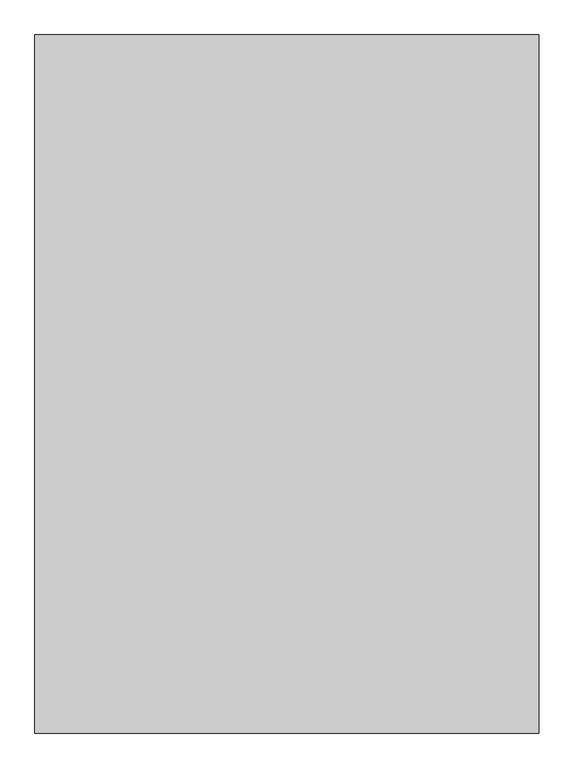
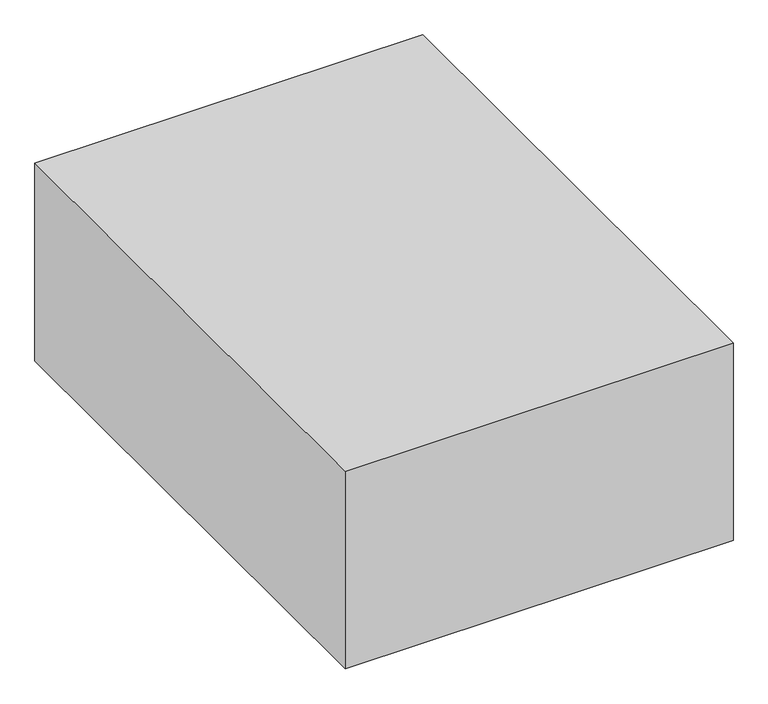
"""IFC4 building model written with IfcOpenShell, lengths in millimetres: proxy geometry, Space Planning Box_hec : Space Planning Box_hec."""

import ifcopenshell
import ifcopenshell.guid

model = None  # the IFC model being written
_history = None  # IfcOwnerHistory: only IFC2X3 demands one
_inside = {}  # id of a spatial element -> (the spatial element, [elements in it])
_under = {}  # id of a project, library or spatial element -> (it, [spatial elements below it])
_declared = {}  # id of a project -> (the project, [libraries it declares])
_typed = {}  # id of a type object -> (the type object, [elements of that type])
_made_of = {}  # id of a material, layer set ... -> (it, [elements and type objects made of it])


def new_model(schema):
    """Start an empty IFC model of exactly this schema.

    Asked for "IFC4X3", IfcOpenShell would pick the latest addendum, in which some entities
    have other attributes; the version numbers below select the first issue.
    IFC2X3 requires an IfcOwnerHistory on every rooted entity: one is made here for all.
    """
    global model, _history
    if schema == "IFC4X3":
        model = ifcopenshell.file(schema_version=(4, 3, 0, 0))
    else:
        model = ifcopenshell.file(schema=schema)
    _inside.clear()
    _under.clear()
    _declared.clear()
    _typed.clear()
    _made_of.clear()
    _history = None
    if model.schema == "IFC2X3":
        org = make("IfcOrganization", Name="unknown")
        user = make(
            "IfcPersonAndOrganization",
            ThePerson=make("IfcPerson", FamilyName="unknown"),
            TheOrganization=org,
        )
        app = make(
            "IfcApplication",
            ApplicationDeveloper=org,
            Version="unknown",
            ApplicationFullName="unknown",
            ApplicationIdentifier="unknown",
        )
        _history = make(
            "IfcOwnerHistory",
            OwningUser=user,
            OwningApplication=app,
            ChangeAction="ADDED",
            CreationDate=0,
        )
    return model


def make(cls, **values):
    """One entity of the class cls with the attributes given. An attribute that is None is left unset."""
    return model.create_entity(
        cls, **{name: value for name, value in values.items() if value is not None}
    )


def rooted(cls, **values):
    """An entity with a GlobalId (a new one), such as an element, a storey or a relation."""
    return make(cls, GlobalId=ifcopenshell.guid.new(), OwnerHistory=_history, **values)


def si_unit(unit_type, name, prefix=None):
    """IfcSIUnit, for example si_unit("LENGTHUNIT", "METRE", prefix="MILLI")."""
    return make("IfcSIUnit", UnitType=unit_type, Prefix=prefix, Name=name)


def assignment(units):
    """IfcUnitAssignment: the units of a project."""
    return None if units is None else make("IfcUnitAssignment", Units=units)


def point(xyz):
    """IfcCartesianPoint."""
    return None if xyz is None else make("IfcCartesianPoint", Coordinates=xyz)


def direction(xyz):
    """IfcDirection."""
    return None if xyz is None else make("IfcDirection", DirectionRatios=xyz)


def frame(location, z_axis=None, x_axis=None):
    """IfcAxis2Placement3D, a coordinate frame: its origin and axes. An axis left out is left unset."""
    return make(
        "IfcAxis2Placement3D",
        Location=point(location),
        Axis=direction(z_axis),
        RefDirection=direction(x_axis),
    )


def origin():
    """The frame at (0, 0, 0) with its axes left unset."""
    return frame((0.0, 0.0, 0.0))


def origin_with_axes():
    """The frame at (0, 0, 0) with the z axis (0, 0, 1) and the x axis (1, 0, 0) written out."""
    return frame((0.0, 0.0, 0.0), z_axis=(0.0, 0.0, 1.0), x_axis=(1.0, 0.0, 0.0))


def place(relative_to, where):
    """IfcLocalPlacement: puts the frame where relative to a parent placement (None: the world)."""
    return make(
        "IfcLocalPlacement", PlacementRelTo=relative_to, RelativePlacement=where
    )


def context(
    kind, dimensions, precision=None, world=None, true_north=None, identifier=None
):
    """IfcGeometricRepresentationContext, for example the 3D "Model" context."""
    return make(
        "IfcGeometricRepresentationContext",
        ContextIdentifier=identifier,
        ContextType=kind,
        CoordinateSpaceDimension=dimensions,
        Precision=precision,
        WorldCoordinateSystem=world,
        TrueNorth=true_north,
    )


def project(units=None, contexts=None):
    """IfcProject with its units and contexts."""
    return rooted(
        "IfcProject",
        Name="project",
        RepresentationContexts=contexts,
        UnitsInContext=assignment(units),
    )


def spatial(cls, under=None, at=None, **own):
    """A site, building, storey or space (cls), placed at a placement, below another one or the project."""
    s = rooted(cls, ObjectPlacement=at, **own)
    if under is not None:
        _under.setdefault(under.id(), (under, []))[1].append(s)
    return s


def polyline(points):
    """IfcPolyline through the points."""
    return make("IfcPolyline", Points=[point(p) for p in points])


def outline(outer, holes=None, kind="AREA"):
    """IfcArbitraryClosedProfileDef: a profile drawn as a closed curve; with holes, ...WithVoids."""
    if holes is None:
        return make("IfcArbitraryClosedProfileDef", ProfileType=kind, OuterCurve=outer)
    return make(
        "IfcArbitraryProfileDefWithVoids",
        ProfileType=kind,
        OuterCurve=outer,
        InnerCurves=holes,
    )


def extrude(swept, where, along, depth):
    """IfcExtrudedAreaSolid: the profile swept, set in the frame where, extruded along a direction by depth."""
    return make(
        "IfcExtrudedAreaSolid",
        SweptArea=swept,
        Position=where,
        ExtrudedDirection=direction(along),
        Depth=depth,
    )


def shape(context_of_items, identifier, shape_type, items):
    """IfcShapeRepresentation: the items that make up one representation, for example the "Body"."""
    return make(
        "IfcShapeRepresentation",
        ContextOfItems=context_of_items,
        RepresentationIdentifier=identifier,
        RepresentationType=shape_type,
        Items=items,
    )


def source(mapping_origin, context_of_items, identifier, shape_type, items):
    """IfcRepresentationMap: a shape defined once, which mapped items show again and again."""
    return make(
        "IfcRepresentationMap",
        MappingOrigin=mapping_origin,
        MappedRepresentation=shape(context_of_items, identifier, shape_type, items),
    )


def transform(
    local_origin,
    x_axis=None,
    y_axis=None,
    z_axis=None,
    scale=None,
    scale2=None,
    scale3=None,
    uniform=True,
):
    """IfcCartesianTransformationOperator3D, or its non-uniform kind. x_axis, y_axis, z_axis: its Axis1, 2, 3."""
    if uniform:
        return make(
            "IfcCartesianTransformationOperator3D",
            Axis1=direction(x_axis),
            Axis2=direction(y_axis),
            LocalOrigin=point(local_origin),
            Scale=scale,
            Axis3=direction(z_axis),
        )
    return make(
        "IfcCartesianTransformationOperator3DnonUniform",
        Axis1=direction(x_axis),
        Axis2=direction(y_axis),
        LocalOrigin=point(local_origin),
        Scale=scale,
        Axis3=direction(z_axis),
        Scale2=scale2,
        Scale3=scale3,
    )


def mapped(mapping_source, mapping_target):
    """IfcMappedItem: shows the shape of a source again, moved by a transform."""
    return make(
        "IfcMappedItem", MappingSource=mapping_source, MappingTarget=mapping_target
    )


def made_of(thing, what):
    """Note that an element or type object is made of a material, layer set ...; save() writes the relation."""
    if what is not None:
        _made_of.setdefault(what.id(), (what, []))[1].append(thing)
    return thing


def element(
    cls,
    number,
    at=None,
    inside=None,
    cuts=None,
    type_object=None,
    material=None,
    context=None,
    identifier="Body",
    shape_type=None,
    held_by="IfcProductDefinitionShape",
    body=None,
    shapes=None,
    **own,
):
    """One element of the class cls, such as IfcWall. Its Tag is "e" and its number.

    at: its placement. inside: the storey or other place that contains it. cuts: it is an
    opening in that element (IfcRelVoidsElement). A single representation is given by context,
    identifier, shape_type and body (its items); several are given by shapes. held_by: the class
    of the entity that holds the representations. save() writes the other relations.
    """
    e = rooted(cls, Tag="e%d" % number, ObjectPlacement=at, **own)
    if body is not None:
        shapes = [shape(context, identifier, shape_type, body)]
    if shapes is not None:
        e.Representation = make(held_by, Representations=shapes)
    if inside is not None:
        _inside.setdefault(inside.id(), (inside, []))[1].append(e)
    if cuts is not None:
        rooted(
            "IfcRelVoidsElement", RelatingBuildingElement=cuts, RelatedOpeningElement=e
        )
    if type_object is not None:
        _typed.setdefault(type_object.id(), (type_object, []))[1].append(e)
    return made_of(e, material)


def aggregate(whole, parts):
    """IfcRelAggregates: a whole, such as a stair, and the parts it consists of."""
    return rooted("IfcRelAggregates", RelatingObject=whole, RelatedObjects=parts)


def save(model, path):
    """Write the relations noted so far, then the file.

    IfcRelAggregates (storeys below a building ...), IfcRelContainedInSpatialStructure (elements
    in a storey), IfcRelDefinesByType, IfcRelAssociatesMaterial and IfcRelDeclares: one each for
    every whole, place, type object, material and project.
    """
    for whole, parts in _under.values():
        aggregate(whole, parts)
    for where, things in _inside.values():
        rooted(
            "IfcRelContainedInSpatialStructure",
            RelatedElements=things,
            RelatingStructure=where,
        )
    for kind, things in _typed.values():
        rooted("IfcRelDefinesByType", RelatedObjects=things, RelatingType=kind)
    for what, things in _made_of.values():
        rooted("IfcRelAssociatesMaterial", RelatedObjects=things, RelatingMaterial=what)
    for by, libraries in _declared.values():
        rooted("IfcRelDeclares", RelatingContext=by, RelatedDefinitions=libraries)
    model.write(path)


def generic_models_5926095e(model_context):
    return source(origin(), model_context, "Body", "SweptSolid", [
        extrude(outline(polyline([(3250.0, 4500.0), (3250.0, -4500.0), (-3250.0, -4500.0), (-3250.0, 4500.0), (3250.0, 4500.0)])), origin_with_axes(), (0.0, 0.0, 1.0), 3500.0),
    ])


if __name__ == "__main__":
    model = new_model("IFC4")
    model_context = context("Model", 3, world=origin())
    ifc_project = project(units=[si_unit("LENGTHUNIT", "METRE", prefix="MILLI")], contexts=[model_context])
    site = spatial("IfcSite", under=ifc_project)
    building = spatial("IfcBuilding", under=site)
    placement = place(None, origin())
    generic_models_shape = generic_models_5926095e(model_context)
    element("IfcBuildingElementProxy", 1, Name="Space Planning Box_hec : Space Planning Box_hec", ObjectType="Space Planning Box_hec : Space Planning Box_hec", at=placement, inside=building, context=model_context, shape_type="MappedRepresentation", body=[
        mapped(generic_models_shape, transform((0.0, 0.0, 0.0), x_axis=(1.0, 0.0, 0.0), y_axis=(0.0, 1.0, 0.0), z_axis=(0.0, 0.0, 1.0))),
    ])
    save(model, "model.ifc")

# Revit data of these elements
# Type "Space Planning Box_hec : Space Planning Box_hec"
#   Type Comments = "..."
#   Room Name [instance default] = "?"
#   Interior Finish [instance default] = ""
#   Exterior Finish [instance default] = ""
#   Department [instance default] = ""
#   Assembly Code = "..."
#   ceiling height [instance default] = 0
#   Width [instance default] = 1524 mm
#   Program Area [instance default] = 0.00 m²
#   Length [instance default] = 1524 mm
#   Height [instance default] = 1524 mm
#   Area [instance default] = 2.32258 m²
#   Fill Color [instance default] = Cyan
#   Default Elevation = 0
# Element 1 (IfcBuildingElementProxy, "Space Planning Box_hec : Space Planning Box_hec")
#   Room Name = "Battery Room"
#   Exterior Finish = "N/A..N/A,,EW2..N/A..N/A"
#   Department = "EL"
#   Width = 6500 mm
#   Program Area = 58.50 m²
#   Length = 9000 mm
#   Height = 3500 mm
#   Area = 58.50 m²
#   Fill Color = Orange
#   Materials on its faces: "Orange"
# Materials
#   "Cyan": class "Generic", colour RGB 0 255 255, transparency 0.2, Cost = 0
#   "Orange": class "Generic", colour RGB 255 165 0, transparency 0.2, Cost = 0
